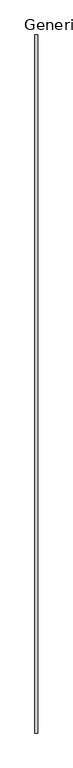
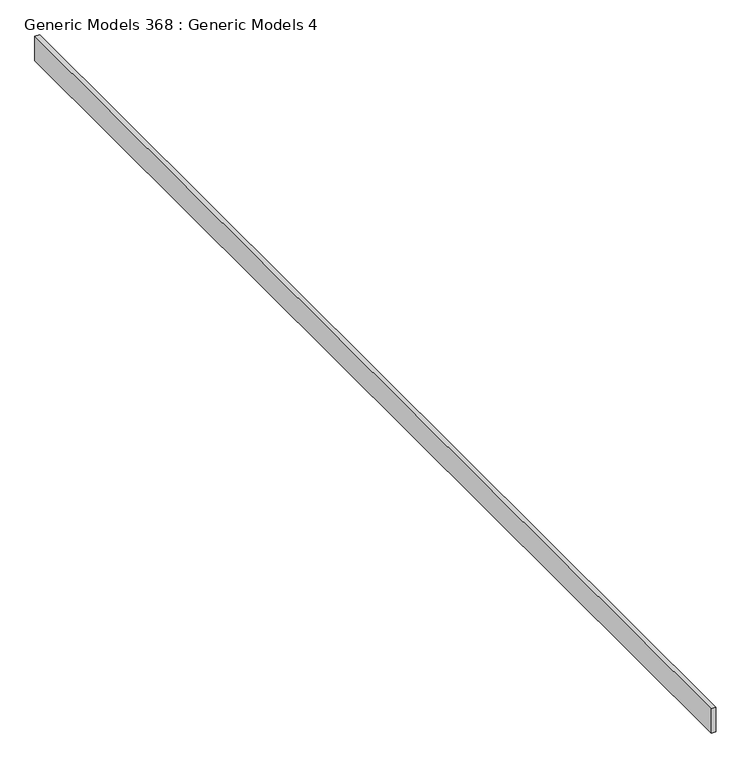
"""IFC4 building model written with IfcOpenShell, lengths in millimetres: proxy geometry, Generic Models 368 : Generic Models 4."""

from ifc_helpers import new_model, si_unit, frame, origin, place, context, project, spatial, polyline, outline, extrude, source, transform, mapped, element, save


def generic_models_368_generic_models_4_51316ca1(model_context):
    return source(origin(), model_context, "Body", "SweptSolid", [
        extrude(outline(polyline([(-6521.6236296, -6864.9230338), (-6547.0236296, -6864.9230338), (-6547.0236296, -464.1230338), (-6521.6236296, -464.1230338), (-6521.6236296, -6864.9230338)])), frame((0.0, 0.0, 129093.3123933), z_axis=(0.0, 0.0, 1.0), x_axis=(1.0, 0.0, 0.0)), (0.0, 0.0, 1.0), 139.7),
    ])


if __name__ == "__main__":
    model = new_model("IFC4")
    model_context = context("Model", 3, world=origin())
    ifc_project = project(units=[si_unit("LENGTHUNIT", "METRE", prefix="MILLI")], contexts=[model_context])
    site = spatial("IfcSite", under=ifc_project)
    building = spatial("IfcBuilding", under=site)
    placement = place(None, origin())
    generic_models_368_generic_models_4_shape = generic_models_368_generic_models_4_51316ca1(model_context)
    element("IfcBuildingElementProxy", 1, Name="Generic Models 368 : Generic Models 4", ObjectType="Generic Models 368 : Generic Models 4", at=placement, inside=building, context=model_context, shape_type="MappedRepresentation", body=[
        mapped(generic_models_368_generic_models_4_shape, transform((0.0, 0.0, 0.0), x_axis=(1.0, 0.0, 0.0), y_axis=(0.0, 1.0, 0.0), z_axis=(0.0, 0.0, 1.0))),
    ])
    save(model, "model.ifc")

# Revit data of these elements
# Element 1 (IfcBuildingElementProxy, "Generic Models 368 : Generic Models 4")
#   Materials on its faces: "_2X BLOCKING AS REQUIRED"
# Materials
#   "_2X BLOCKING AS REQUIRED": class "Generic", colour RGB 177 130 114, transparency 0, Cost = 0
